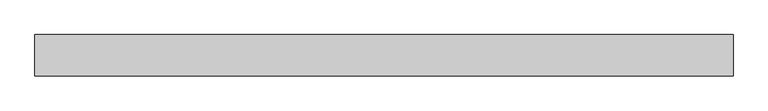
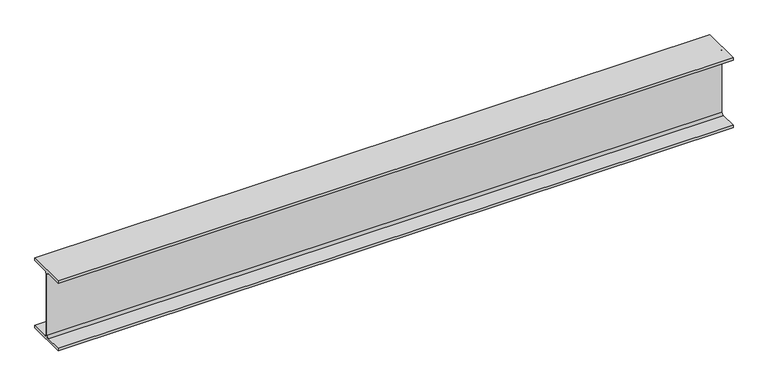
"""IFC4 building model written with IfcOpenShell, lengths in millimetres: beam geometry, Steel Beam_H-KSD3502 : H_SB_ASB_H-250x125x6x9."""

import ifcopenshell
import ifcopenshell.guid

model = None  # the IFC model being written
_history = None  # IfcOwnerHistory: only IFC2X3 demands one
_inside = {}  # id of a spatial element -> (the spatial element, [elements in it])
_under = {}  # id of a project, library or spatial element -> (it, [spatial elements below it])
_declared = {}  # id of a project -> (the project, [libraries it declares])
_typed = {}  # id of a type object -> (the type object, [elements of that type])
_made_of = {}  # id of a material, layer set ... -> (it, [elements and type objects made of it])


def new_model(schema):
    """Start an empty IFC model of exactly this schema.

    Asked for "IFC4X3", IfcOpenShell would pick the latest addendum, in which some entities
    have other attributes; the version numbers below select the first issue.
    IFC2X3 requires an IfcOwnerHistory on every rooted entity: one is made here for all.
    """
    global model, _history
    if schema == "IFC4X3":
        model = ifcopenshell.file(schema_version=(4, 3, 0, 0))
    else:
        model = ifcopenshell.file(schema=schema)
    _inside.clear()
    _under.clear()
    _declared.clear()
    _typed.clear()
    _made_of.clear()
    _history = None
    if model.schema == "IFC2X3":
        org = make("IfcOrganization", Name="unknown")
        user = make(
            "IfcPersonAndOrganization",
            ThePerson=make("IfcPerson", FamilyName="unknown"),
            TheOrganization=org,
        )
        app = make(
            "IfcApplication",
            ApplicationDeveloper=org,
            Version="unknown",
            ApplicationFullName="unknown",
            ApplicationIdentifier="unknown",
        )
        _history = make(
            "IfcOwnerHistory",
            OwningUser=user,
            OwningApplication=app,
            ChangeAction="ADDED",
            CreationDate=0,
        )
    return model


def make(cls, **values):
    """One entity of the class cls with the attributes given. An attribute that is None is left unset."""
    return model.create_entity(
        cls, **{name: value for name, value in values.items() if value is not None}
    )


def rooted(cls, **values):
    """An entity with a GlobalId (a new one), such as an element, a storey or a relation."""
    return make(cls, GlobalId=ifcopenshell.guid.new(), OwnerHistory=_history, **values)


def si_unit(unit_type, name, prefix=None):
    """IfcSIUnit, for example si_unit("LENGTHUNIT", "METRE", prefix="MILLI")."""
    return make("IfcSIUnit", UnitType=unit_type, Prefix=prefix, Name=name)


def assignment(units):
    """IfcUnitAssignment: the units of a project."""
    return None if units is None else make("IfcUnitAssignment", Units=units)


def point(xyz):
    """IfcCartesianPoint."""
    return None if xyz is None else make("IfcCartesianPoint", Coordinates=xyz)


def direction(xyz):
    """IfcDirection."""
    return None if xyz is None else make("IfcDirection", DirectionRatios=xyz)


def frame(location, z_axis=None, x_axis=None):
    """IfcAxis2Placement3D, a coordinate frame: its origin and axes. An axis left out is left unset."""
    return make(
        "IfcAxis2Placement3D",
        Location=point(location),
        Axis=direction(z_axis),
        RefDirection=direction(x_axis),
    )


def frame_2d(location, x_axis=None):
    """IfcAxis2Placement2D, a coordinate frame in the plane: its origin and x axis."""
    return make(
        "IfcAxis2Placement2D", Location=point(location), RefDirection=direction(x_axis)
    )


def origin():
    """The frame at (0, 0, 0) with its axes left unset."""
    return frame((0.0, 0.0, 0.0))


def place(relative_to, where):
    """IfcLocalPlacement: puts the frame where relative to a parent placement (None: the world)."""
    return make(
        "IfcLocalPlacement", PlacementRelTo=relative_to, RelativePlacement=where
    )


def context(
    kind, dimensions, precision=None, world=None, true_north=None, identifier=None
):
    """IfcGeometricRepresentationContext, for example the 3D "Model" context."""
    return make(
        "IfcGeometricRepresentationContext",
        ContextIdentifier=identifier,
        ContextType=kind,
        CoordinateSpaceDimension=dimensions,
        Precision=precision,
        WorldCoordinateSystem=world,
        TrueNorth=true_north,
    )


def project(units=None, contexts=None):
    """IfcProject with its units and contexts."""
    return rooted(
        "IfcProject",
        Name="project",
        RepresentationContexts=contexts,
        UnitsInContext=assignment(units),
    )


def spatial(cls, under=None, at=None, **own):
    """A site, building, storey or space (cls), placed at a placement, below another one or the project."""
    s = rooted(cls, ObjectPlacement=at, **own)
    if under is not None:
        _under.setdefault(under.id(), (under, []))[1].append(s)
    return s


def polyline(points):
    """IfcPolyline through the points."""
    return make("IfcPolyline", Points=[point(p) for p in points])


def circle_curve(where, radius):
    """IfcCircle in the frame where."""
    return make("IfcCircle", Position=where, Radius=radius)


def trimmed(basis, trim1, trim2, sense, master):
    """IfcTrimmedCurve: the piece of a basis curve between two trims."""
    return make(
        "IfcTrimmedCurve",
        BasisCurve=basis,
        Trim1=trim1,
        Trim2=trim2,
        SenseAgreement=sense,
        MasterRepresentation=master,
    )


def segment(curve, same_sense, transition):
    """IfcCompositeCurveSegment."""
    return make(
        "IfcCompositeCurveSegment",
        Transition=transition,
        SameSense=same_sense,
        ParentCurve=curve,
    )


def composite_curve(segments, self_intersect=None):
    """IfcCompositeCurve: segments joined end to end."""
    return make("IfcCompositeCurve", Segments=segments, SelfIntersect=self_intersect)


def outline(outer, holes=None, kind="AREA"):
    """IfcArbitraryClosedProfileDef: a profile drawn as a closed curve; with holes, ...WithVoids."""
    if holes is None:
        return make("IfcArbitraryClosedProfileDef", ProfileType=kind, OuterCurve=outer)
    return make(
        "IfcArbitraryProfileDefWithVoids",
        ProfileType=kind,
        OuterCurve=outer,
        InnerCurves=holes,
    )


def extrude(swept, where, along, depth):
    """IfcExtrudedAreaSolid: the profile swept, set in the frame where, extruded along a direction by depth."""
    return make(
        "IfcExtrudedAreaSolid",
        SweptArea=swept,
        Position=where,
        ExtrudedDirection=direction(along),
        Depth=depth,
    )


def shape(context_of_items, identifier, shape_type, items):
    """IfcShapeRepresentation: the items that make up one representation, for example the "Body"."""
    return make(
        "IfcShapeRepresentation",
        ContextOfItems=context_of_items,
        RepresentationIdentifier=identifier,
        RepresentationType=shape_type,
        Items=items,
    )


def source(mapping_origin, context_of_items, identifier, shape_type, items):
    """IfcRepresentationMap: a shape defined once, which mapped items show again and again."""
    return make(
        "IfcRepresentationMap",
        MappingOrigin=mapping_origin,
        MappedRepresentation=shape(context_of_items, identifier, shape_type, items),
    )


def transform(
    local_origin,
    x_axis=None,
    y_axis=None,
    z_axis=None,
    scale=None,
    scale2=None,
    scale3=None,
    uniform=True,
):
    """IfcCartesianTransformationOperator3D, or its non-uniform kind. x_axis, y_axis, z_axis: its Axis1, 2, 3."""
    if uniform:
        return make(
            "IfcCartesianTransformationOperator3D",
            Axis1=direction(x_axis),
            Axis2=direction(y_axis),
            LocalOrigin=point(local_origin),
            Scale=scale,
            Axis3=direction(z_axis),
        )
    return make(
        "IfcCartesianTransformationOperator3DnonUniform",
        Axis1=direction(x_axis),
        Axis2=direction(y_axis),
        LocalOrigin=point(local_origin),
        Scale=scale,
        Axis3=direction(z_axis),
        Scale2=scale2,
        Scale3=scale3,
    )


def mapped(mapping_source, mapping_target):
    """IfcMappedItem: shows the shape of a source again, moved by a transform."""
    return make(
        "IfcMappedItem", MappingSource=mapping_source, MappingTarget=mapping_target
    )


def made_of(thing, what):
    """Note that an element or type object is made of a material, layer set ...; save() writes the relation."""
    if what is not None:
        _made_of.setdefault(what.id(), (what, []))[1].append(thing)
    return thing


def element(
    cls,
    number,
    at=None,
    inside=None,
    cuts=None,
    type_object=None,
    material=None,
    context=None,
    identifier="Body",
    shape_type=None,
    held_by="IfcProductDefinitionShape",
    body=None,
    shapes=None,
    **own,
):
    """One element of the class cls, such as IfcWall. Its Tag is "e" and its number.

    at: its placement. inside: the storey or other place that contains it. cuts: it is an
    opening in that element (IfcRelVoidsElement). A single representation is given by context,
    identifier, shape_type and body (its items); several are given by shapes. held_by: the class
    of the entity that holds the representations. save() writes the other relations.
    """
    e = rooted(cls, Tag="e%d" % number, ObjectPlacement=at, **own)
    if body is not None:
        shapes = [shape(context, identifier, shape_type, body)]
    if shapes is not None:
        e.Representation = make(held_by, Representations=shapes)
    if inside is not None:
        _inside.setdefault(inside.id(), (inside, []))[1].append(e)
    if cuts is not None:
        rooted(
            "IfcRelVoidsElement", RelatingBuildingElement=cuts, RelatedOpeningElement=e
        )
    if type_object is not None:
        _typed.setdefault(type_object.id(), (type_object, []))[1].append(e)
    return made_of(e, material)


def aggregate(whole, parts):
    """IfcRelAggregates: a whole, such as a stair, and the parts it consists of."""
    return rooted("IfcRelAggregates", RelatingObject=whole, RelatedObjects=parts)


def save(model, path):
    """Write the relations noted so far, then the file.

    IfcRelAggregates (storeys below a building ...), IfcRelContainedInSpatialStructure (elements
    in a storey), IfcRelDefinesByType, IfcRelAssociatesMaterial and IfcRelDeclares: one each for
    every whole, place, type object, material and project.
    """
    for whole, parts in _under.values():
        aggregate(whole, parts)
    for where, things in _inside.values():
        rooted(
            "IfcRelContainedInSpatialStructure",
            RelatedElements=things,
            RelatingStructure=where,
        )
    for kind, things in _typed.values():
        rooted("IfcRelDefinesByType", RelatedObjects=things, RelatingType=kind)
    for what, things in _made_of.values():
        rooted("IfcRelAssociatesMaterial", RelatedObjects=things, RelatingMaterial=what)
    for by, libraries in _declared.values():
        rooted("IfcRelDeclares", RelatingContext=by, RelatedDefinitions=libraries)
    model.write(path)


def beam_a866aaba(model_context):
    return source(origin(), model_context, "Body", "SweptSolid", [
        extrude(outline(composite_curve([segment(polyline([(82.5, -141.5), (82.5, -151.7), (-82.5, -151.7), (-82.5, -141.5), (-11.9, -141.5)]), True, "CONTINUOUS"), segment(trimmed(circle_curve(frame_2d((-11.9, -132.6)), 8.9), [point((-11.9, -141.5))], [point((-3.0, -132.6))], True, "CARTESIAN"), True, "CONTINUOUS"), segment(polyline([(-3.0, -132.6), (-3.0, 132.6)]), True, "CONTINUOUS"), segment(trimmed(circle_curve(frame_2d((-11.9, 132.6)), 8.9), [point((-3.0, 132.6))], [point((-11.9, 141.5))], True, "CARTESIAN"), True, "CONTINUOUS"), segment(polyline([(-11.9, 141.5), (-82.5, 141.5), (-82.5, 151.7), (82.5, 151.7), (82.5, 141.5), (11.9, 141.5)]), True, "CONTINUOUS"), segment(trimmed(circle_curve(frame_2d((11.9, 132.6)), 8.9), [point((11.9, 141.5))], [point((3.0, 132.6))], True, "CARTESIAN"), True, "CONTINUOUS"), segment(polyline([(3.0, 132.6), (3.0, -132.6)]), True, "CONTINUOUS"), segment(trimmed(circle_curve(frame_2d((11.9, -132.6)), 8.9), [point((3.0, -132.6))], [point((11.9, -141.5))], True, "CARTESIAN"), True, "CONTINUOUS"), segment(polyline([(11.9, -141.5), (82.5, -141.5)]), True, "CONTINUOUS")], self_intersect=False)), frame((-1387.3, 0.0, 0.0), z_axis=(1.0, 0.0, 0.0), x_axis=(0.0, 1.0, 0.0)), (0.0, 0.0, 1.0), 2774.6),
    ])


if __name__ == "__main__":
    model = new_model("IFC4")
    model_context = context("Model", 3, world=origin())
    ifc_project = project(units=[si_unit("LENGTHUNIT", "METRE", prefix="MILLI")], contexts=[model_context])
    site = spatial("IfcSite", under=ifc_project)
    building = spatial("IfcBuilding", under=site)
    placement = place(None, origin())
    beam_shape = beam_a866aaba(model_context)
    element("IfcBeam", 1, ObjectType="Steel Beam_H-KSD3502 : H_SB_ASB_H-250x125x6x9", at=placement, inside=building, context=model_context, shape_type="MappedRepresentation", body=[
        mapped(beam_shape, transform((0.0, 0.0, 0.0), x_axis=(1.0, 0.0, 0.0), y_axis=(0.0, 1.0, 0.0), z_axis=(0.0, 0.0, 1.0))),
    ])
    save(model, "model.ifc")

# Revit data of these elements
# Type "Steel Beam_H-KSD3502 : H_SB_ASB_H-250x125x6x9"
#   Width = 12.5 cm
#   Web Thickness = 0.6 cm
#   Web Fillet = 1.2 cm
#   Warping Constant = 42539.8 cm⁶
#   Torsional Moment of Inertia = 7.8102 cm⁴
#   Torsional Modulus = 1.0 cm³
#   Section Area = 37.66 cm²
#   Plastic Modulus weak axis = 73.1 cm³
#   Plastic Modulus strong axis = 366.0 cm³
#   Perimeter = 0.97 m²/m
#   Nominal Weight = 29.60 kgf/m
#   Moment of Inertia weak axis = 294.00 cm⁴
#   Moment of Inertia strong axis = 4050.00 cm⁴
#   Height = 25.0 cm
#   Flange Thickness = 0.9 cm
#   Elastic Modulus weak axis = 47.0 cm³
#   Elastic Modulus strong axis = 324.0 cm³
#   Centroid Vertical = 12.5 cm
#   Centroid Horizontal = 6.25 cm
#   Length [instance default] = 1.5240 m
#   Structural Material [instance default] = Steel, 45-345
#   Assembly Code = ""
# Element 1 (IfcBeam, "Steel Beam_H-KSD3502 : H_SB_ASB_H-250x125x6x9")
#   Structural Material = none
# Materials
#   "Steel, 45-345": class "Metal", colour RGB 189 187 185, transparency 0, Description = "Steel 345 MPa", Cost = 0
